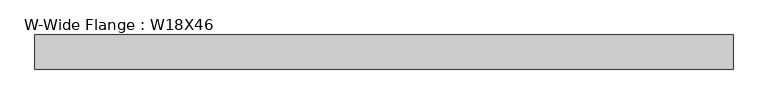
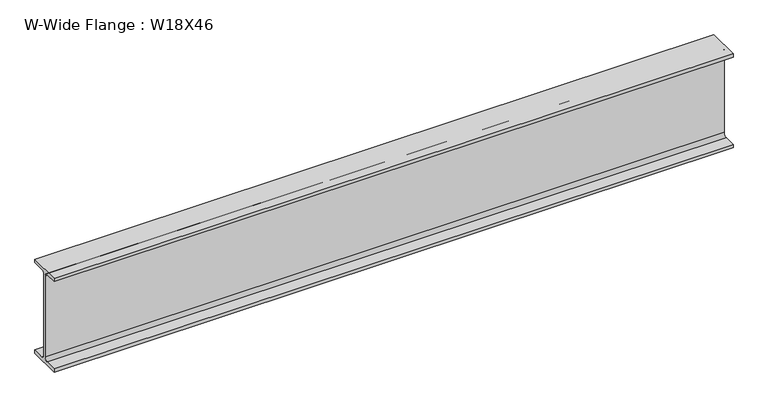
"""IFC4 building model written with IfcOpenShell, lengths in millimetres: beam geometry, W-Wide Flange : W18X46."""

from ifc_helpers import new_model, si_unit, point, frame, frame_2d, origin, place, context, project, spatial, polyline, circle_curve, trimmed, segment, composite_curve, outline, extrude, source, transform, mapped, element, save


def w_wide_flange_w18x46_42f80e1e(model_context):
    return source(origin(), model_context, "Body", "SweptSolid", [
        extrude(outline(composite_curve([segment(polyline([(76.962, -214.503), (76.962, -229.87), (-76.962, -229.87), (-76.962, -214.503), (-20.955, -214.503)]), True, "CONTINUOUS"), segment(trimmed(circle_curve(frame_2d((-20.955, -198.12)), 16.383), [point((-20.955, -214.503))], [point((-4.572, -198.12))], True, "CARTESIAN"), True, "CONTINUOUS"), segment(polyline([(-4.572, -198.12), (-4.572, 198.12)]), True, "CONTINUOUS"), segment(trimmed(circle_curve(frame_2d((-20.955, 198.12)), 16.383), [point((-4.572, 198.12))], [point((-20.955, 214.503))], True, "CARTESIAN"), True, "CONTINUOUS"), segment(polyline([(-20.955, 214.503), (-76.962, 214.503), (-76.962, 229.87), (76.962, 229.87), (76.962, 214.503), (20.955, 214.503)]), True, "CONTINUOUS"), segment(trimmed(circle_curve(frame_2d((20.955, 198.12)), 16.383), [point((20.955, 214.503))], [point((4.572, 198.12))], True, "CARTESIAN"), True, "CONTINUOUS"), segment(polyline([(4.572, 198.12), (4.572, -198.12)]), True, "CONTINUOUS"), segment(trimmed(circle_curve(frame_2d((20.955, -198.12)), 16.383), [point((4.572, -198.12))], [point((20.955, -214.503))], True, "CARTESIAN"), True, "CONTINUOUS"), segment(polyline([(20.955, -214.503), (76.962, -214.503)]), True, "CONTINUOUS")], self_intersect=False)), frame((-1574.8, 0.0, 0.0), z_axis=(1.0, 0.0, 0.0), x_axis=(0.0, 1.0, 0.0)), (0.0, 0.0, 1.0), 3149.6),
    ])


if __name__ == "__main__":
    model = new_model("IFC4")
    model_context = context("Model", 3, world=origin())
    ifc_project = project(units=[si_unit("LENGTHUNIT", "METRE", prefix="MILLI")], contexts=[model_context])
    site = spatial("IfcSite", under=ifc_project)
    building = spatial("IfcBuilding", under=site)
    placement = place(None, origin())
    w_wide_flange_w18x46_shape = w_wide_flange_w18x46_42f80e1e(model_context)
    element("IfcBeam", 1, ObjectType="W-Wide Flange : W18X46", at=placement, inside=building, context=model_context, shape_type="MappedRepresentation", body=[
        mapped(w_wide_flange_w18x46_shape, transform((0.0, 0.0, 0.0), x_axis=(1.0, 0.0, 0.0), y_axis=(0.0, 1.0, 0.0), z_axis=(0.0, 0.0, 1.0))),
    ])
    save(model, "model.ifc")

# Revit data of these elements
# Type "W-Wide Flange : W18X46"
#   Assembly Code = "B10"
#   W = 46
#   Length [instance default] = 5' - 0"
#   bf = 0' - 6.06"
#   d = 1' - 6.1"
#   k = 0' - 1 1/4"
#   k2 = 0' - 0.645"
#   tf = 0' - 0.605"
#   tw = 0' - 0.36"
#   A = 0.09375 SF
#   Structural Material [instance default] = Steel ASTM A992
# Element 1 (IfcBeam, "W-Wide Flange : W18X46")
#   Materials on its faces: "Steel ASTM A992"
# Materials
#   "Steel ASTM A992": class "Metal", colour RGB 199 199 199, transparency 0, Description = "Structural steel 50ksi", Cost = 0
